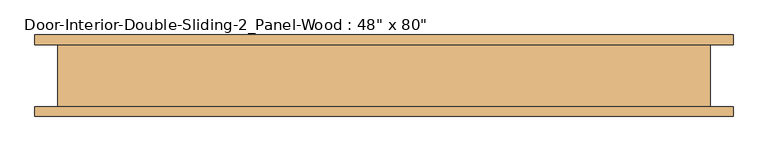
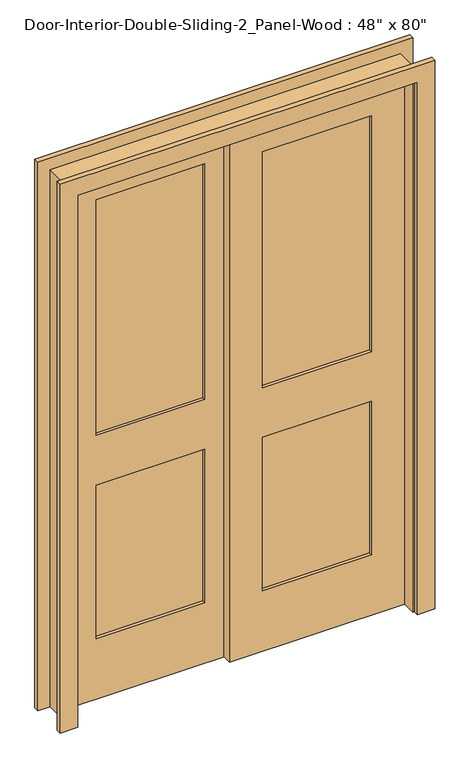
"""IFC4 building model written with IfcOpenShell, lengths in millimetres: door geometry."""

from ifc_helpers import new_model, si_unit, frame, origin, place, context, project, spatial, polyline, outline, extrude, source, transform, mapped, element, save


def door_5e6fa93e(model_context):
    return source(origin(), model_context, "Body", "SweptSolid", [
        extrude(outline(polyline([(488.95, -1.0583333), (95.25, -1.0583333), (95.25, 10.5833333), (488.95, 10.5833333), (488.95, -1.0583333)])), frame((0.0, 0.0, 1009.65), z_axis=(0.0, 0.0, 1.0), x_axis=(1.0, 0.0, 0.0)), (0.0, 0.0, 1.0), 903.2875),
        extrude(outline(polyline([(488.95, -1.0583333), (95.25, -1.0583333), (95.25, 10.5833333), (488.95, 10.5833333), (488.95, -1.0583333)])), frame((0.0, 0.0, 231.775), z_axis=(0.0, 0.0, 1.0), x_axis=(1.0, 0.0, 0.0)), (0.0, 0.0, 1.0), 587.375),
        extrude(outline(polyline([(2032.0, -25.4), (0.0, -25.4), (0.0, 609.6), (2032.0, 609.6), (2032.0, -25.4)]), holes=[polyline([(1912.9375, 95.25), (1912.9375, 488.95), (1009.65, 488.95), (1009.65, 95.25), (1912.9375, 95.25)]), polyline([(819.15, 95.25), (819.15, 488.95), (231.775, 488.95), (231.775, 95.25), (819.15, 95.25)])]), frame((0.0, -12.7, 0.0), z_axis=(0.0, 1.0, 0.0), x_axis=(0.0, 0.0, 1.0)), (0.0, 0.0, 1.0), 34.925),
        extrude(outline(polyline([(-95.25, 33.8666667), (-488.95, 33.8666667), (-488.95, 45.5083333), (-95.25, 45.5083333), (-95.25, 33.8666667)])), frame((0.0, 0.0, 1009.65), z_axis=(0.0, 0.0, 1.0), x_axis=(1.0, 0.0, 0.0)), (0.0, 0.0, 1.0), 903.2875),
        extrude(outline(polyline([(-95.25, 33.8666667), (-488.95, 33.8666667), (-488.95, 45.5083333), (-95.25, 45.5083333), (-95.25, 33.8666667)])), frame((0.0, 0.0, 231.775), z_axis=(0.0, 0.0, 1.0), x_axis=(1.0, 0.0, 0.0)), (0.0, 0.0, 1.0), 587.375),
        extrude(outline(polyline([(2032.0, -609.6), (0.0, -609.6), (0.0, 25.4), (2032.0, 25.4), (2032.0, -609.6)]), holes=[polyline([(1912.9375, -488.95), (1912.9375, -95.25), (1009.65, -95.25), (1009.65, -488.95), (1912.9375, -488.95)]), polyline([(819.15, -488.95), (819.15, -95.25), (231.775, -95.25), (231.775, -488.95), (819.15, -488.95)])]), frame((0.0, 22.225, 0.0), z_axis=(0.0, 1.0, 0.0), x_axis=(0.0, 0.0, 1.0)), (0.0, 0.0, 1.0), 34.925),
        extrude(outline(polyline([(0.0, 609.6), (0.0, 635.0), (2057.4, 635.0), (2057.4, -635.0), (0.0, -635.0), (0.0, -609.6), (2032.0, -609.6), (2032.0, 609.6), (0.0, 609.6)])), frame((0.0, -63.5, 0.0), z_axis=(0.0, 1.0, 0.0), x_axis=(0.0, 0.0, 1.0)), (0.0, 0.0, 1.0), 120.65),
        extrude(outline(polyline([(0.0, 615.95), (0.0, 679.45), (2101.85, 679.45), (2101.85, -679.45), (0.0, -679.45), (0.0, -615.95), (2038.35, -615.95), (2038.35, 615.95), (0.0, 615.95)])), frame((0.0, -82.55, 0.0), z_axis=(0.0, 1.0, 0.0), x_axis=(0.0, 0.0, 1.0)), (0.0, 0.0, 1.0), 19.05),
        extrude(outline(polyline([(0.0, 615.95), (0.0, 679.45), (2101.85, 679.45), (2101.85, -679.45), (0.0, -679.45), (0.0, -615.95), (2038.35, -615.95), (2038.35, 615.95), (0.0, 615.95)])), frame((0.0, 57.15, 0.0), z_axis=(0.0, 1.0, 0.0), x_axis=(0.0, 0.0, 1.0)), (0.0, 0.0, 1.0), 19.05),
    ])


if __name__ == "__main__":
    model = new_model("IFC4")
    model_context = context("Model", 3, world=origin())
    ifc_project = project(units=[si_unit("LENGTHUNIT", "METRE", prefix="MILLI")], contexts=[model_context])
    site = spatial("IfcSite", under=ifc_project)
    building = spatial("IfcBuilding", under=site)
    placement = place(None, origin())
    door_shape = door_5e6fa93e(model_context)
    element("IfcDoor", 1, ObjectType="Door-Interior-Double-Sliding-2_Panel-Wood : 48\" x 80\"", at=placement, inside=building, context=model_context, shape_type="MappedRepresentation", body=[
        mapped(door_shape, transform((0.0, 0.0, 0.0), x_axis=(1.0, 0.0, 0.0), y_axis=(0.0, 1.0, 0.0), z_axis=(0.0, 0.0, 1.0))),
    ])
    save(model, "model.ifc")

# Revit data of these elements
# Type "Door-Interior-Double-Sliding-2_Panel-Wood : 48\" x 80\""
#   Type Mark = "22"
#   Assembly Code = "C1020300"
#   Analytic Construction = "Wooden"
#   Top Rail = 0' - 4 11/16"
#   Thickness = 0' - 1 3/8"
#   Thermal Resistance (R) = 2.5876 (h·ft²·°F)/BTU
#   Stiles = 0' - 4 3/4"
#   Rough Width = 4' - 2"
#   Rough Height = 6' - 9"
#   Lock Rail = 0' - 7 1/2"
#   Height = 6' - 8"
#   Width = 4' - 0"
#   Heat Transfer Coefficient (U) = 0.3865 BTU/(h·ft²·°F)
#   Bottom Rail = 0' - 9 1/8"
#   Trim Material = Cherry
#   Panel Material = Cherry
#   Frame Material = Cherry
#   Visual Light Transmittance = 0
#   Solar Heat Gain Coefficient = 0
#   Wall Closure = (empty or 0)
#   Function = (empty or 0)
# Element 1 (IfcDoor, "Door-Interior-Double-Sliding-2_Panel-Wood : 48\" x 80\"")
#   Materials on its faces: "Cherry"
# Materials
#   "Cherry": class "Wood", colour RGB 226 177 128, transparency 0, Description = "Prunus Serotina", Cost = 0
